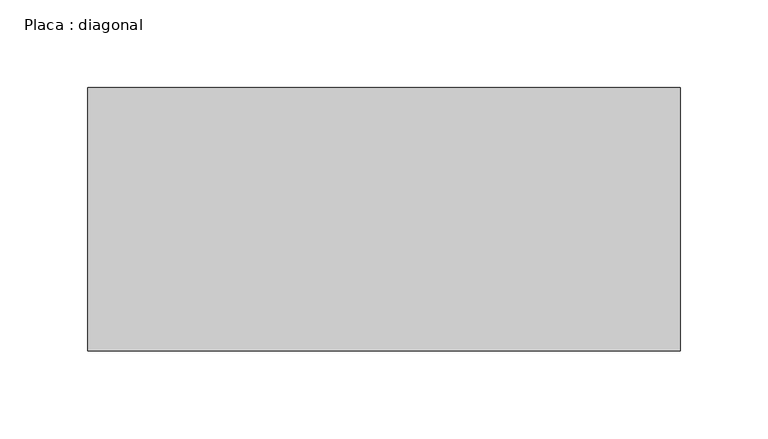
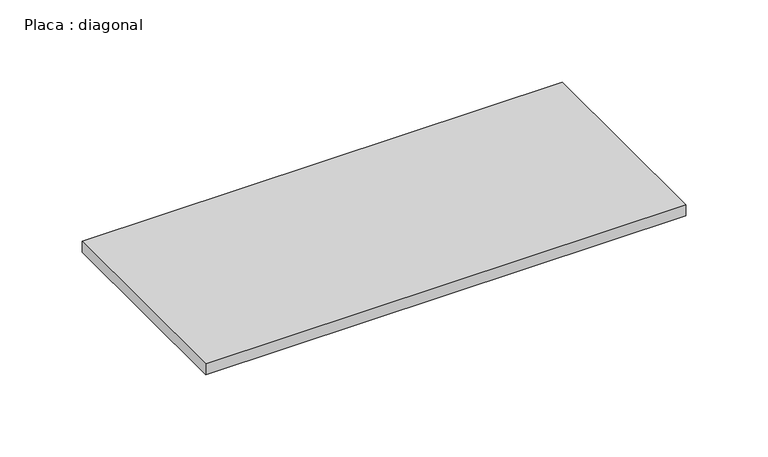
"""IFC4 building model written with IfcOpenShell, lengths in millimetres: beam geometry, Placa : diagonal."""

from ifc_helpers import new_model, si_unit, frame, origin, place, context, project, spatial, polyline, outline, extrude, source, transform, mapped, element, save


def placa_diagonal_d8887dd5(model_context):
    return source(origin(), model_context, "Body", "SweptSolid", [
        extrude(outline(polyline([(168.6204805, 75.0), (168.6204805, -75.0), (-168.6204805, -75.0), (-168.6204805, 75.0), (168.6204805, 75.0)])), frame((0.0, 0.0, -4.0), z_axis=(0.0, 0.0, 1.0), x_axis=(1.0, 0.0, 0.0)), (0.0, 0.0, 1.0), 8.0),
    ])


if __name__ == "__main__":
    model = new_model("IFC4")
    model_context = context("Model", 3, world=origin())
    ifc_project = project(units=[si_unit("LENGTHUNIT", "METRE", prefix="MILLI")], contexts=[model_context])
    site = spatial("IfcSite", under=ifc_project)
    building = spatial("IfcBuilding", under=site)
    placement = place(None, origin())
    placa_diagonal_shape = placa_diagonal_d8887dd5(model_context)
    element("IfcBeam", 1, ObjectType="Placa : diagonal", at=placement, inside=building, context=model_context, shape_type="MappedRepresentation", body=[
        mapped(placa_diagonal_shape, transform((0.0, 0.0, 0.0), x_axis=(1.0, 0.0, 0.0), y_axis=(0.0, 1.0, 0.0), z_axis=(0.0, 0.0, 1.0))),
    ])
    save(model, "model.ifc")

# Revit data of these elements
# Type "Placa : diagonal"
#   W = 0
#   Length [instance default] = 1.50 m
#   b = 0.15 m
#   d = 0.008 m
#   A = 0 m²
#   Structural Material [instance default] = Aço, 45-345
# Element 1 (IfcBeam, "Placa : diagonal")
#   Materials on its faces: "Aço, 45-345"
# Materials
#   "Aço, 45-345": class "Metal", colour RGB 247 247 247, transparency 0, Description = "Aço 345 MPa", Cost = 0
